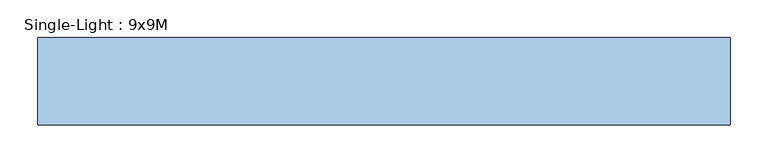
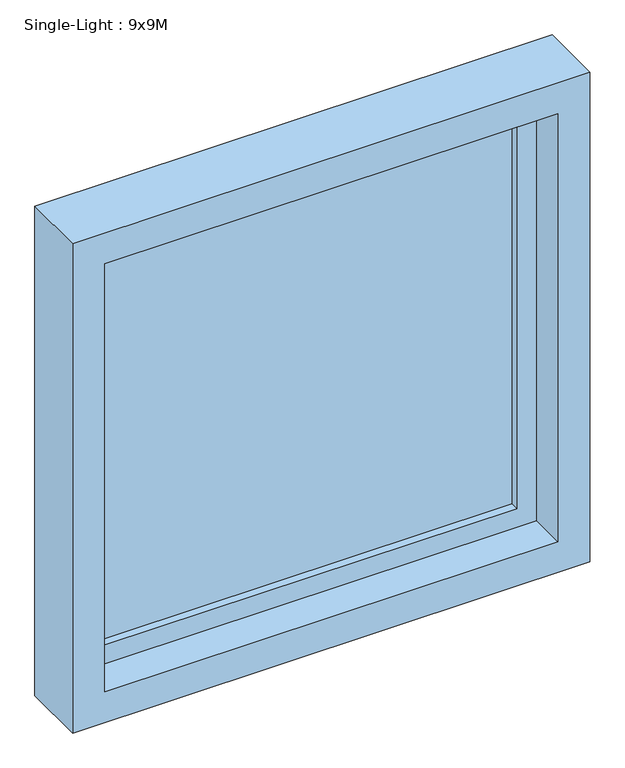
"""IFC4 building model written with IfcOpenShell, lengths in millimetres: window geometry, Single-Light : 9x9M."""

from ifc_helpers import new_model, si_unit, frame, origin, place, context, project, spatial, polyline, outline, extrude, faceted_brep, source, transform, mapped, element, save


def single_light_9x9m_9d4aa27d(model_context):
    return source(origin(), model_context, "Body", "SolidModel", [
        extrude(outline(polyline([(1670.0, -414.0), (842.0, -414.0), (842.0, 414.0), (1670.0, 414.0), (1670.0, -414.0)]), holes=[polyline([(1620.0, 364.0), (892.0, 364.0), (892.0, -364.0), (1620.0, -364.0), (1620.0, 364.0)])]), frame((0.0, 134.0, 0.0), z_axis=(0.0, 1.0, 0.0), x_axis=(0.0, 0.0, 1.0)), (0.0, 0.0, 1.0), 50.0),
        faceted_brep([(-456.0, 69.0, 800.0), (-456.0, 184.0, 800.0), (456.0, 184.0, 800.0), (456.0, 69.0, 800.0), (456.0, 184.0, 1712.0), (456.0, 69.0, 1712.0), (-456.0, 184.0, 1712.0), (414.0, 184.0, 1670.0), (-414.0, 184.0, 1670.0), (-414.0, 184.0, 842.0), (414.0, 184.0, 842.0), (-456.0, 69.0, 1712.0), (399.0, 69.0, 857.0), (-399.0, 69.0, 857.0), (-399.0, 69.0, 1655.0), (399.0, 69.0, 1655.0), (-399.0, 134.0, 857.0), (399.0, 134.0, 857.0), (399.0, 134.0, 1655.0), (414.0, 134.0, 842.0), (-414.0, 134.0, 842.0), (-414.0, 134.0, 1670.0), (414.0, 134.0, 1670.0), (-399.0, 134.0, 1655.0)], [[[0, 1, 2, 3]], [[3, 2, 4, 5]], [[2, 1, 6, 4], [7, 8, 9, 10]], [[5, 11, 0, 3], [12, 13, 14, 15]], [[16, 13, 12, 17]], [[17, 12, 15, 18]], [[19, 20, 21, 22], [18, 23, 16, 17]], [[9, 20, 19, 10]], [[10, 19, 22, 7]], [[11, 6, 1, 0]], [[23, 14, 13, 16]], [[8, 21, 20, 9]], [[5, 4, 6, 11]], [[18, 15, 14, 23]], [[7, 22, 21, 8]]]),
        extrude(outline(polyline([(-364.0, 170.0), (364.0, 170.0), (364.0, 148.0), (-364.0, 148.0), (-364.0, 170.0)])), frame((0.0, 0.0, 892.0), z_axis=(0.0, 0.0, 1.0), x_axis=(1.0, 0.0, 0.0)), (0.0, 0.0, 1.0), 728.0),
    ])


if __name__ == "__main__":
    model = new_model("IFC4")
    model_context = context("Model", 3, world=origin())
    ifc_project = project(units=[si_unit("LENGTHUNIT", "METRE", prefix="MILLI")], contexts=[model_context])
    site = spatial("IfcSite", under=ifc_project)
    building = spatial("IfcBuilding", under=site)
    placement = place(None, origin())
    single_light_9x9m_shape = single_light_9x9m_9d4aa27d(model_context)
    element("IfcWindow", 1, ObjectType="Single-Light : 9x9M", at=placement, inside=building, context=model_context, shape_type="MappedRepresentation", body=[
        mapped(single_light_9x9m_shape, transform((0.0, 0.0, 0.0), x_axis=(1.0, 0.0, 0.0), y_axis=(0.0, 1.0, 0.0), z_axis=(0.0, 0.0, 1.0))),
    ])
    save(model, "model.ifc")

# Revit data of these elements
# Type "Single-Light : 9x9M"
#   Type Mark = "44"
#   Creator Organization [instance default] = "© Danish Educational Content"
#   Creator Name [instance default] = "© Erik Falck Jørgensen"
#   Creator Build [instance default] = "2017.0801.0"
#   Analytic Construction = "<None>"
#   length#5 = -36 mm
#   length#4 = -14 mm
#   length#3 = 120 mm
#   length#2 = 57 mm
#   length#1 = 0 mm
#   Seal Width = 12 mm
#   Rough Width = 912 mm
#   Rough Height = 912 mm
#   Rebate Depth = 50 mm
#   Rabbet Width = 15 mm
#   Rabbet Depth = 50 mm
#   Height = 888 mm
#   Glass Thickness = 22 mm
#   Frame Width = 50 mm
#   Frame Depth = 50 mm
#   Exterior Direction [instance default] = 0.00°
#   Case Depth = 115 mm
#   Case Width = 45 mm
#   Default Sill Height = 800 mm
#   Width = 888 mm
#   Sealing = no
#   Hinging = yes
#   Wall Closure = 1
#   Above Cutplane [instance default] = no
#   Wall Surface = none
#   Sill Plate = none
#   Glass = none
#   Frame/Mullion = none
#   Embrasure = none
#   Case/Transom = none
# Element 1 (IfcWindow, "Single-Light : 9x9M")
#   Materials on its faces: "Default Frame/Mullion (Interior/Exterior)", "Glass"
# Materials
#   "Default Frame/Mullion (Interior/Exterior)": class "Generic", colour RGB 205 205 205, transparency 0, Description = "Udefineret karm/ramme materiale", Cost = 0
#   "Glass": class "Glass", colour RGB 180 200 255, transparency 0.75, Description = "Generisk glas", Cost = 0
